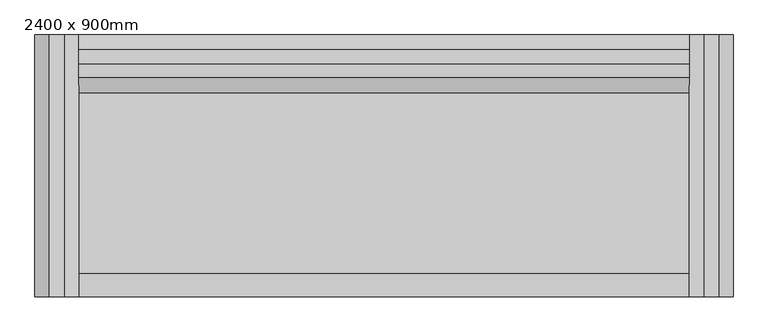
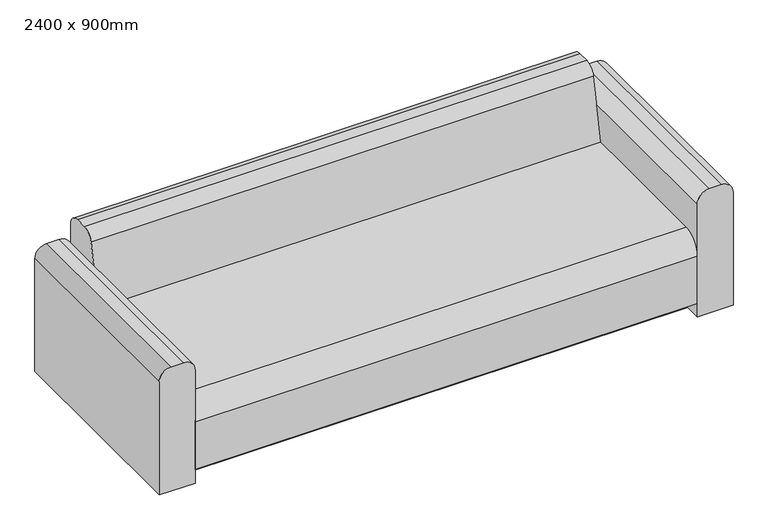
"""IFC4 building model written with IfcOpenShell, lengths in millimetres: furniture geometry, ソファ－I型 : 2400 x 900mm."""

from ifc_helpers import new_model, si_unit, point, frame, frame_2d, origin, place, context, project, spatial, polyline, circle_curve, trimmed, segment, composite_curve, outline, extrude, source, transform, mapped, element, save


def furniture_2400_x_900mm_2d6eb021(model_context):
    return source(origin(), model_context, "Body", "SweptSolid", [
        extrude(outline(composite_curve([segment(trimmed(circle_curve(frame_2d((500.0, -1150.0)), 50.0), [point((550.0, -1150.0))], [point((500.0, -1200.0))], False, "CARTESIAN"), True, "CONTINUOUS"), segment(polyline([(500.0, -1200.0), (0.0, -1200.0), (0.0, -1050.0), (500.0, -1050.0)]), True, "CONTINUOUS"), segment(trimmed(circle_curve(frame_2d((500.0, -1100.0)), 50.0), [point((500.0, -1050.0))], [point((550.0, -1100.0))], False, "CARTESIAN"), True, "CONTINUOUS"), segment(polyline([(550.0, -1100.0), (550.0, -1150.0)]), True, "CONTINUOUS")], self_intersect=False)), frame((0.0, -450.0, 0.0), z_axis=(0.0, 1.0, 0.0), x_axis=(0.0, 0.0, 1.0)), (0.0, 0.0, 1.0), 900.0),
        extrude(outline(composite_curve([segment(polyline([(550.0, 1150.0), (550.0, 1100.0)]), True, "CONTINUOUS"), segment(trimmed(circle_curve(frame_2d((500.0, 1100.0)), 50.0), [point((550.0, 1100.0))], [point((500.0, 1050.0))], False, "CARTESIAN"), True, "CONTINUOUS"), segment(polyline([(500.0, 1050.0), (0.0, 1050.0), (0.0, 1200.0), (500.0, 1200.0)]), True, "CONTINUOUS"), segment(trimmed(circle_curve(frame_2d((500.0, 1150.0)), 50.0), [point((500.0, 1200.0))], [point((550.0, 1150.0))], False, "CARTESIAN"), True, "CONTINUOUS")], self_intersect=False)), frame((0.0, -450.0, 0.0), z_axis=(0.0, 1.0, 0.0), x_axis=(0.0, 0.0, 1.0)), (0.0, 0.0, 1.0), 900.0),
        extrude(outline(composite_curve([segment(trimmed(circle_curve(frame_2d((350.9901951, 600.0)), 50.0), [point((301.9611614, 609.8058068))], [point((350.9901951, 650.0))], False, "CARTESIAN"), True, "CONTINUOUS"), segment(polyline([(350.9901951, 650.0), (400.0, 650.0)]), True, "CONTINUOUS"), segment(trimmed(circle_curve(frame_2d((400.0, 600.0)), 50.0), [point((400.0, 650.0))], [point((450.0, 600.0))], False, "CARTESIAN"), True, "CONTINUOUS"), segment(polyline([(450.0, 600.0), (450.0, 0.0), (-380.0, 0.0), (-380.0, 60.0), (-450.0, 60.0), (-450.0, 270.0)]), True, "CONTINUOUS"), segment(trimmed(circle_curve(frame_2d((-370.0, 270.0)), 80.0), [point((-450.0, 270.0))], [point((-370.0, 350.0))], False, "CARTESIAN"), True, "CONTINUOUS"), segment(polyline([(-370.0, 350.0), (250.0, 350.0), (301.9611614, 609.8058068)]), True, "CONTINUOUS")], self_intersect=False)), frame((-1050.0, 0.0, 0.0), z_axis=(1.0, 0.0, 0.0), x_axis=(0.0, 1.0, 0.0)), (0.0, 0.0, 1.0), 2100.0),
    ])


if __name__ == "__main__":
    model = new_model("IFC4")
    model_context = context("Model", 3, world=origin())
    ifc_project = project(units=[si_unit("LENGTHUNIT", "METRE", prefix="MILLI")], contexts=[model_context])
    site = spatial("IfcSite", under=ifc_project)
    building = spatial("IfcBuilding", under=site)
    placement = place(None, origin())
    furniture_2400_x_900mm_shape = furniture_2400_x_900mm_2d6eb021(model_context)
    element("IfcFurniture", 1, ObjectType="ソファ－I型 : 2400 x 900mm", at=placement, inside=building, context=model_context, shape_type="MappedRepresentation", body=[
        mapped(furniture_2400_x_900mm_shape, transform((0.0, 0.0, 0.0), x_axis=(1.0, 0.0, 0.0), y_axis=(0.0, 1.0, 0.0), z_axis=(0.0, 0.0, 1.0))),
    ])
    save(model, "model.ifc")

# Revit data of these elements
# Project information
#   プロジェクト発行日 = "発行日"
#   プロジェクト ステータス = "プロジェクト ステータス"
#   クライアント名 = "オーナ"
#   計画地住所 = "ここにアドレスを入力"
#   プロジェクト名 = "プロジェクト名"
#   プロジェクト番号 = "0001"
# Type "ソファ－I型 : 2400 x 900mm"
#   Keynote = "12490.Y1"
#   座面高さ = 350 mm
#   幅 = 2400 mm
#   奥行き = 900 mm
#   本体 = モチアミ - 無地 - グレー
#   Default Elevation = 0
# Element 1 (IfcFurniture, "ソファ－I型 : 2400 x 900mm")
#   Materials on its faces: "モチアミ - 無地 - グレー"
# Materials
#   "モチアミ - 無地 - グレー": class "モチアミ", colour RGB 65 63 65, transparency 0, Cost = 0
